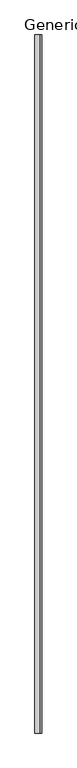
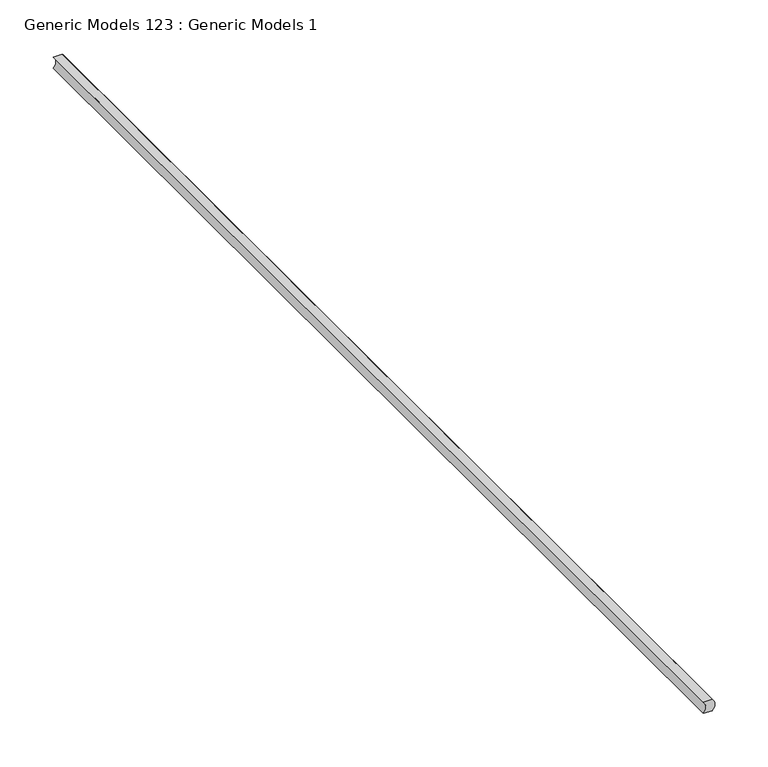
"""IFC4 building model written with IfcOpenShell, lengths in millimetres: proxy geometry, Generic Models 123 : Generic Models 1."""

from ifc_helpers import new_model, si_unit, point, frame, frame_2d, origin, place, context, project, spatial, polyline, circle_curve, trimmed, segment, composite_curve, outline, extrude, source, transform, mapped, element, save


def generic_models_123_generic_models_1_084f7e48(model_context):
    return source(origin(), model_context, "Body", "SweptSolid", [
        extrude(outline(composite_curve([segment(polyline([(2438.4, 48444.15), (2438.4, 48453.675)]), True, "CONTINUOUS"), segment(trimmed(circle_curve(frame_2d((2444.75, 48447.845519)), 8.620055), [point((2438.4, 48453.675))], [point((2451.1, 48453.675))], False, "CARTESIAN"), True, "CONTINUOUS"), segment(polyline([(2451.1, 48453.675), (2451.1, 48444.15)]), True, "CONTINUOUS"), segment(trimmed(circle_curve(frame_2d((2444.75, 48438.320519)), 8.620055), [point((2451.1, 48444.15))], [point((2438.4, 48444.15))], True, "CARTESIAN"), True, "CONTINUOUS")], self_intersect=False)), frame((0.0, 0.0, 0.0), z_axis=(0.0, 1.0, 0.0), x_axis=(0.0, 0.0, 1.0)), (0.0, 0.0, 1.0), 1219.2),
    ])


if __name__ == "__main__":
    model = new_model("IFC4")
    model_context = context("Model", 3, world=origin())
    ifc_project = project(units=[si_unit("LENGTHUNIT", "METRE", prefix="MILLI")], contexts=[model_context])
    site = spatial("IfcSite", under=ifc_project)
    building = spatial("IfcBuilding", under=site)
    placement = place(None, origin())
    generic_models_123_generic_models_1_shape = generic_models_123_generic_models_1_084f7e48(model_context)
    element("IfcBuildingElementProxy", 1, Name="Generic Models 123 : Generic Models 1", ObjectType="Generic Models 123 : Generic Models 1", at=placement, inside=building, context=model_context, shape_type="MappedRepresentation", body=[
        mapped(generic_models_123_generic_models_1_shape, transform((0.0, 0.0, 0.0), x_axis=(1.0, 0.0, 0.0), y_axis=(0.0, 1.0, 0.0), z_axis=(0.0, 0.0, 1.0))),
    ])
    save(model, "model.ifc")

# Revit data of these elements
# Element 1 (IfcBuildingElementProxy, "Generic Models 123 : Generic Models 1")
#   Materials on its faces: "ACOUSTICAL SEALANT"
# Materials
#   "ACOUSTICAL SEALANT": class "Unassigned", colour RGB 120 120 120, transparency 0, Cost = 0
